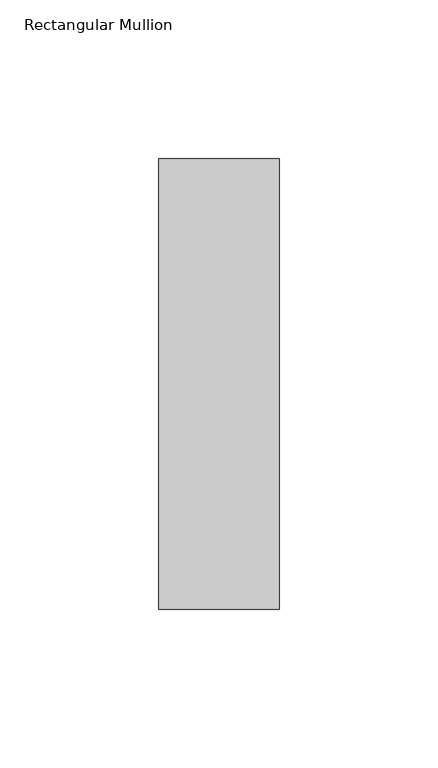
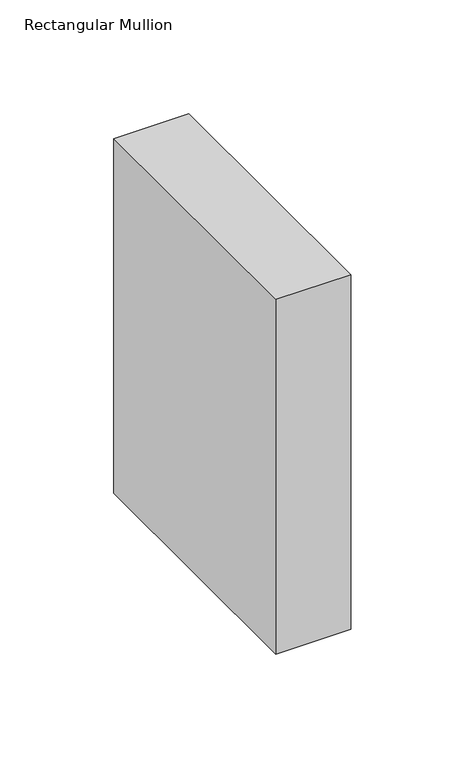
"""IFC4 building model written with IfcOpenShell, lengths in millimetres: member geometry, Rectangular Mullion : NLRS_21_CWM_hsb-regel 38x142_gen_rsf."""

from ifc_helpers import new_model, si_unit, frame, origin, place, context, project, spatial, polyline, outline, extrude, source, transform, mapped, element, save


def rectangular_mullion_50c5102b(model_context):
    return source(origin(), model_context, "Body", "SweptSolid", [
        extrude(outline(polyline([(0.0, -71.0), (-38.0, -71.0), (-38.0, 71.0), (0.0, 71.0), (0.0, -71.0)])), frame((0.0, 0.0, -189.9999997), z_axis=(0.0, 0.0, 1.0), x_axis=(1.0, 0.0, 0.0)), (0.0, 0.0, 1.0), 189.9999997),
    ])


if __name__ == "__main__":
    model = new_model("IFC4")
    model_context = context("Model", 3, world=origin())
    ifc_project = project(units=[si_unit("LENGTHUNIT", "METRE", prefix="MILLI")], contexts=[model_context])
    site = spatial("IfcSite", under=ifc_project)
    building = spatial("IfcBuilding", under=site)
    placement = place(None, origin())
    rectangular_mullion_shape = rectangular_mullion_50c5102b(model_context)
    element("IfcMember", 1, ObjectType="Rectangular Mullion : NLRS_21_CWM_hsb-regel 38x142_gen_rsf", at=placement, inside=building, context=model_context, shape_type="MappedRepresentation", body=[
        mapped(rectangular_mullion_shape, transform((0.0, 0.0, 0.0), x_axis=(1.0, 0.0, 0.0), y_axis=(0.0, 1.0, 0.0), z_axis=(0.0, 0.0, 1.0))),
    ])
    save(model, "model.ifc")

# Revit data of these elements
# Type "Rectangular Mullion : NLRS_21_CWM_hsb-regel 38x142_gen_rsf"
#   Export Type to IFC As = "IfcWall"
#   Type IfcGUID = "07M7mRoiH1CR8m_RSKIwpF"
#   Assembly Code = "21.10"
#   built-in parameter 1007322 = 0.465879 (stored number, unit not read)
#   built-in parameter 1007321 = 0.062336 (stored number, unit not read)
#   built-in parameter 1007320 = 0.062336 (stored number, unit not read)
# Element 1 (IfcMember, "Rectangular Mullion : NLRS_21_CWM_hsb-regel 38x142_gen_rsf")
#   Materials on its faces: "NLRS_i2_hout naaldhout vuren_gen_rsf"
# Materials
#   "NLRS_i2_hout naaldhout vuren_gen_rsf": class "I - Hout", colour RGB 234 199 147, transparency 0, Keynote = "i2", Manufacturer = "Revit Standards Foundation", URL = "www.revitstandards.org", Description = "hout vuren", Cost = 0
